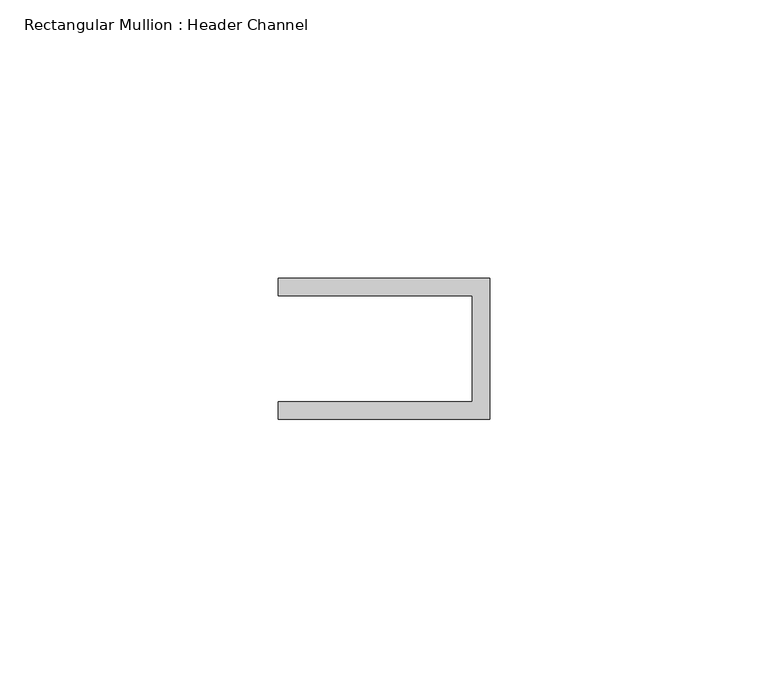
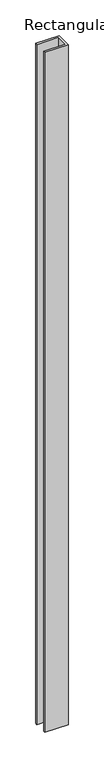
"""IFC4 building model written with IfcOpenShell, lengths in millimetres: member geometry, Rectangular Mullion : Header Channel."""

from ifc_helpers import new_model, si_unit, frame, origin, place, context, project, spatial, polyline, outline, extrude, source, transform, mapped, element, save


def rectangular_mullion_header_channel_550d867f(model_context):
    return source(origin(), model_context, "Body", "SweptSolid", [
        extrude(outline(polyline([(0.0, -12.7), (-38.1, -12.7), (-38.1, -9.525), (-3.175, -9.525), (-3.175, 9.525), (-38.1, 9.525), (-38.1, 12.7), (0.0, 12.7), (0.0, -12.7)])), frame((0.0, 0.0, -1165.225), z_axis=(0.0, 0.0, 1.0), x_axis=(1.0, 0.0, 0.0)), (0.0, 0.0, 1.0), 1165.225),
    ])


if __name__ == "__main__":
    model = new_model("IFC4")
    model_context = context("Model", 3, world=origin())
    ifc_project = project(units=[si_unit("LENGTHUNIT", "METRE", prefix="MILLI")], contexts=[model_context])
    site = spatial("IfcSite", under=ifc_project)
    building = spatial("IfcBuilding", under=site)
    placement = place(None, origin())
    rectangular_mullion_header_channel_shape = rectangular_mullion_header_channel_550d867f(model_context)
    element("IfcMember", 1, ObjectType="Rectangular Mullion : Header Channel", at=placement, inside=building, context=model_context, shape_type="MappedRepresentation", body=[
        mapped(rectangular_mullion_header_channel_shape, transform((0.0, 0.0, 0.0), x_axis=(1.0, 0.0, 0.0), y_axis=(0.0, 1.0, 0.0), z_axis=(0.0, 0.0, 1.0))),
    ])
    save(model, "model.ifc")

# Revit data of these elements
# Type "Rectangular Mullion : Header Channel"
#   built-in parameter 1007322 = 0.0833333 (stored number, unit not read)
#   built-in parameter 1007321 = -0.03125 (stored number, unit not read)
#   built-in parameter 1007320 = 0.0416667 (stored number, unit not read)
# Element 1 (IfcMember, "Rectangular Mullion : Header Channel")
#   Materials on its faces: "ALUM"
# Materials
#   "ALUM": class "Generic", colour RGB 157 157 157, transparency 0, Cost = 0
